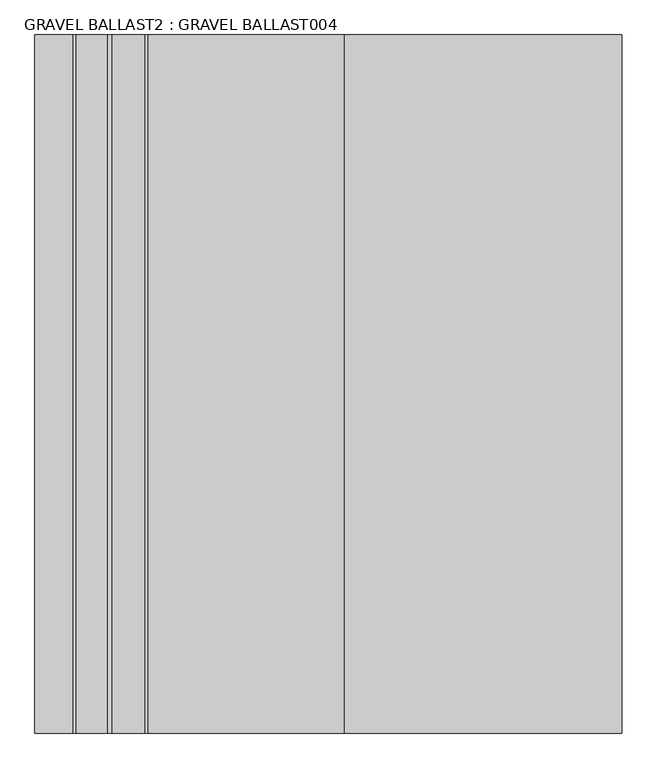
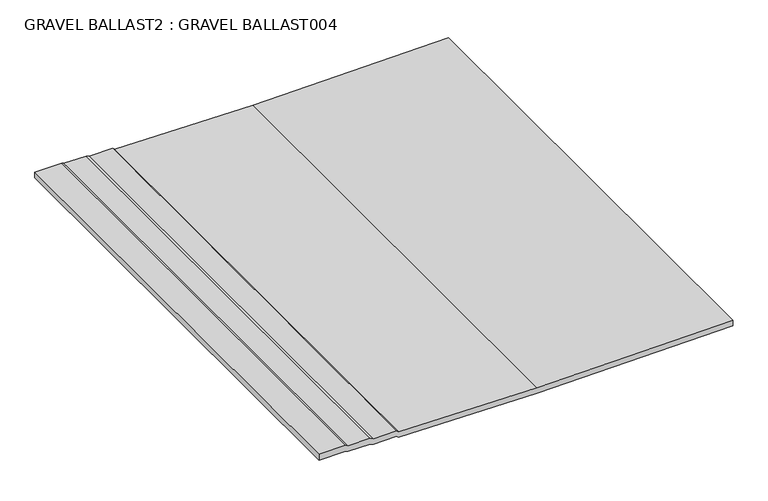
"""IFC4 building model written with IfcOpenShell, lengths in millimetres: proxy geometry, GRAVEL BALLAST2 : GRAVEL BALLAST004."""

import ifcopenshell
import ifcopenshell.guid

model = None  # the IFC model being written
_history = None  # IfcOwnerHistory: only IFC2X3 demands one
_inside = {}  # id of a spatial element -> (the spatial element, [elements in it])
_under = {}  # id of a project, library or spatial element -> (it, [spatial elements below it])
_declared = {}  # id of a project -> (the project, [libraries it declares])
_typed = {}  # id of a type object -> (the type object, [elements of that type])
_made_of = {}  # id of a material, layer set ... -> (it, [elements and type objects made of it])


def new_model(schema):
    """Start an empty IFC model of exactly this schema.

    Asked for "IFC4X3", IfcOpenShell would pick the latest addendum, in which some entities
    have other attributes; the version numbers below select the first issue.
    IFC2X3 requires an IfcOwnerHistory on every rooted entity: one is made here for all.
    """
    global model, _history
    if schema == "IFC4X3":
        model = ifcopenshell.file(schema_version=(4, 3, 0, 0))
    else:
        model = ifcopenshell.file(schema=schema)
    _inside.clear()
    _under.clear()
    _declared.clear()
    _typed.clear()
    _made_of.clear()
    _history = None
    if model.schema == "IFC2X3":
        org = make("IfcOrganization", Name="unknown")
        user = make(
            "IfcPersonAndOrganization",
            ThePerson=make("IfcPerson", FamilyName="unknown"),
            TheOrganization=org,
        )
        app = make(
            "IfcApplication",
            ApplicationDeveloper=org,
            Version="unknown",
            ApplicationFullName="unknown",
            ApplicationIdentifier="unknown",
        )
        _history = make(
            "IfcOwnerHistory",
            OwningUser=user,
            OwningApplication=app,
            ChangeAction="ADDED",
            CreationDate=0,
        )
    return model


def make(cls, **values):
    """One entity of the class cls with the attributes given. An attribute that is None is left unset."""
    return model.create_entity(
        cls, **{name: value for name, value in values.items() if value is not None}
    )


def rooted(cls, **values):
    """An entity with a GlobalId (a new one), such as an element, a storey or a relation."""
    return make(cls, GlobalId=ifcopenshell.guid.new(), OwnerHistory=_history, **values)


def si_unit(unit_type, name, prefix=None):
    """IfcSIUnit, for example si_unit("LENGTHUNIT", "METRE", prefix="MILLI")."""
    return make("IfcSIUnit", UnitType=unit_type, Prefix=prefix, Name=name)


def assignment(units):
    """IfcUnitAssignment: the units of a project."""
    return None if units is None else make("IfcUnitAssignment", Units=units)


def point(xyz):
    """IfcCartesianPoint."""
    return None if xyz is None else make("IfcCartesianPoint", Coordinates=xyz)


def direction(xyz):
    """IfcDirection."""
    return None if xyz is None else make("IfcDirection", DirectionRatios=xyz)


def frame(location, z_axis=None, x_axis=None):
    """IfcAxis2Placement3D, a coordinate frame: its origin and axes. An axis left out is left unset."""
    return make(
        "IfcAxis2Placement3D",
        Location=point(location),
        Axis=direction(z_axis),
        RefDirection=direction(x_axis),
    )


def origin():
    """The frame at (0, 0, 0) with its axes left unset."""
    return frame((0.0, 0.0, 0.0))


def place(relative_to, where):
    """IfcLocalPlacement: puts the frame where relative to a parent placement (None: the world)."""
    return make(
        "IfcLocalPlacement", PlacementRelTo=relative_to, RelativePlacement=where
    )


def context(
    kind, dimensions, precision=None, world=None, true_north=None, identifier=None
):
    """IfcGeometricRepresentationContext, for example the 3D "Model" context."""
    return make(
        "IfcGeometricRepresentationContext",
        ContextIdentifier=identifier,
        ContextType=kind,
        CoordinateSpaceDimension=dimensions,
        Precision=precision,
        WorldCoordinateSystem=world,
        TrueNorth=true_north,
    )


def project(units=None, contexts=None):
    """IfcProject with its units and contexts."""
    return rooted(
        "IfcProject",
        Name="project",
        RepresentationContexts=contexts,
        UnitsInContext=assignment(units),
    )


def spatial(cls, under=None, at=None, **own):
    """A site, building, storey or space (cls), placed at a placement, below another one or the project."""
    s = rooted(cls, ObjectPlacement=at, **own)
    if under is not None:
        _under.setdefault(under.id(), (under, []))[1].append(s)
    return s


def polyline(points):
    """IfcPolyline through the points."""
    return make("IfcPolyline", Points=[point(p) for p in points])


def outline(outer, holes=None, kind="AREA"):
    """IfcArbitraryClosedProfileDef: a profile drawn as a closed curve; with holes, ...WithVoids."""
    if holes is None:
        return make("IfcArbitraryClosedProfileDef", ProfileType=kind, OuterCurve=outer)
    return make(
        "IfcArbitraryProfileDefWithVoids",
        ProfileType=kind,
        OuterCurve=outer,
        InnerCurves=holes,
    )


def extrude(swept, where, along, depth):
    """IfcExtrudedAreaSolid: the profile swept, set in the frame where, extruded along a direction by depth."""
    return make(
        "IfcExtrudedAreaSolid",
        SweptArea=swept,
        Position=where,
        ExtrudedDirection=direction(along),
        Depth=depth,
    )


def shape(context_of_items, identifier, shape_type, items):
    """IfcShapeRepresentation: the items that make up one representation, for example the "Body"."""
    return make(
        "IfcShapeRepresentation",
        ContextOfItems=context_of_items,
        RepresentationIdentifier=identifier,
        RepresentationType=shape_type,
        Items=items,
    )


def source(mapping_origin, context_of_items, identifier, shape_type, items):
    """IfcRepresentationMap: a shape defined once, which mapped items show again and again."""
    return make(
        "IfcRepresentationMap",
        MappingOrigin=mapping_origin,
        MappedRepresentation=shape(context_of_items, identifier, shape_type, items),
    )


def transform(
    local_origin,
    x_axis=None,
    y_axis=None,
    z_axis=None,
    scale=None,
    scale2=None,
    scale3=None,
    uniform=True,
):
    """IfcCartesianTransformationOperator3D, or its non-uniform kind. x_axis, y_axis, z_axis: its Axis1, 2, 3."""
    if uniform:
        return make(
            "IfcCartesianTransformationOperator3D",
            Axis1=direction(x_axis),
            Axis2=direction(y_axis),
            LocalOrigin=point(local_origin),
            Scale=scale,
            Axis3=direction(z_axis),
        )
    return make(
        "IfcCartesianTransformationOperator3DnonUniform",
        Axis1=direction(x_axis),
        Axis2=direction(y_axis),
        LocalOrigin=point(local_origin),
        Scale=scale,
        Axis3=direction(z_axis),
        Scale2=scale2,
        Scale3=scale3,
    )


def mapped(mapping_source, mapping_target):
    """IfcMappedItem: shows the shape of a source again, moved by a transform."""
    return make(
        "IfcMappedItem", MappingSource=mapping_source, MappingTarget=mapping_target
    )


def made_of(thing, what):
    """Note that an element or type object is made of a material, layer set ...; save() writes the relation."""
    if what is not None:
        _made_of.setdefault(what.id(), (what, []))[1].append(thing)
    return thing


def element(
    cls,
    number,
    at=None,
    inside=None,
    cuts=None,
    type_object=None,
    material=None,
    context=None,
    identifier="Body",
    shape_type=None,
    held_by="IfcProductDefinitionShape",
    body=None,
    shapes=None,
    **own,
):
    """One element of the class cls, such as IfcWall. Its Tag is "e" and its number.

    at: its placement. inside: the storey or other place that contains it. cuts: it is an
    opening in that element (IfcRelVoidsElement). A single representation is given by context,
    identifier, shape_type and body (its items); several are given by shapes. held_by: the class
    of the entity that holds the representations. save() writes the other relations.
    """
    e = rooted(cls, Tag="e%d" % number, ObjectPlacement=at, **own)
    if body is not None:
        shapes = [shape(context, identifier, shape_type, body)]
    if shapes is not None:
        e.Representation = make(held_by, Representations=shapes)
    if inside is not None:
        _inside.setdefault(inside.id(), (inside, []))[1].append(e)
    if cuts is not None:
        rooted(
            "IfcRelVoidsElement", RelatingBuildingElement=cuts, RelatedOpeningElement=e
        )
    if type_object is not None:
        _typed.setdefault(type_object.id(), (type_object, []))[1].append(e)
    return made_of(e, material)


def aggregate(whole, parts):
    """IfcRelAggregates: a whole, such as a stair, and the parts it consists of."""
    return rooted("IfcRelAggregates", RelatingObject=whole, RelatedObjects=parts)


def save(model, path):
    """Write the relations noted so far, then the file.

    IfcRelAggregates (storeys below a building ...), IfcRelContainedInSpatialStructure (elements
    in a storey), IfcRelDefinesByType, IfcRelAssociatesMaterial and IfcRelDeclares: one each for
    every whole, place, type object, material and project.
    """
    for whole, parts in _under.values():
        aggregate(whole, parts)
    for where, things in _inside.values():
        rooted(
            "IfcRelContainedInSpatialStructure",
            RelatedElements=things,
            RelatingStructure=where,
        )
    for kind, things in _typed.values():
        rooted("IfcRelDefinesByType", RelatedObjects=things, RelatingType=kind)
    for what, things in _made_of.values():
        rooted("IfcRelAssociatesMaterial", RelatedObjects=things, RelatingMaterial=what)
    for by, libraries in _declared.values():
        rooted("IfcRelDeclares", RelatingContext=by, RelatedDefinitions=libraries)
    model.write(path)


def gravel_ballast2_gravel_ballast004_1e64bb1d(model_context):
    return source(origin(), model_context, "Body", "SweptSolid", [
        extrude(outline(polyline([(40274.2359465, -2672.3662777), (40269.9546965, -2663.6558285), (40269.9546965, -2573.0689144), (40264.2272344, -2560.2242751), (40265.8726651, -2466.2725277), (40258.4625089, -2457.9990902), (40250.2437589, -1894.9286556), (40261.546875, -1099.1907959), (40286.2851563, -1099.1907959), (40274.9820403, -1894.9286556), (40283.2007903, -2457.9990902), (40290.6109465, -2466.2725277), (40288.9655158, -2560.2242751), (40294.6929777, -2573.0689144), (40294.6929777, -2663.6558285), (40298.9742278, -2672.3662777), (40298.9742278, -2781.8657894), (40274.2359465, -2781.8657894), (40274.2359465, -2672.3662777)])), frame((0.0, 1000.0, 0.0), z_axis=(0.0, 1.0, 0.0), x_axis=(0.0, 0.0, 1.0)), (0.0, 0.0, 1.0), 2000.0),
    ])


if __name__ == "__main__":
    model = new_model("IFC4")
    model_context = context("Model", 3, world=origin())
    ifc_project = project(units=[si_unit("LENGTHUNIT", "METRE", prefix="MILLI")], contexts=[model_context])
    site = spatial("IfcSite", under=ifc_project)
    building = spatial("IfcBuilding", under=site)
    placement = place(None, origin())
    gravel_ballast2_gravel_ballast004_shape = gravel_ballast2_gravel_ballast004_1e64bb1d(model_context)
    element("IfcBuildingElementProxy", 1, Name="GRAVEL BALLAST2 : GRAVEL BALLAST004", ObjectType="GRAVEL BALLAST2 : GRAVEL BALLAST004", at=placement, inside=building, context=model_context, shape_type="MappedRepresentation", body=[
        mapped(gravel_ballast2_gravel_ballast004_shape, transform((0.0, 0.0, 0.0), x_axis=(1.0, 0.0, 0.0), y_axis=(0.0, 1.0, 0.0), z_axis=(0.0, 0.0, 1.0))),
    ])
    save(model, "model.ifc")

# Revit data of these elements
# Type "GRAVEL BALLAST2 : GRAVEL BALLAST004"
#   NameOverride = "GRAVEL BALLAST004"
# Element 1 (IfcBuildingElementProxy, "GRAVEL BALLAST2 : GRAVEL BALLAST004")
#   Materials on its faces: "GRAVEL BALLAST"
# Materials
#   "GRAVEL BALLAST": class "Unassigned", colour RGB 128 128 128, transparency 0, Cost = 0
